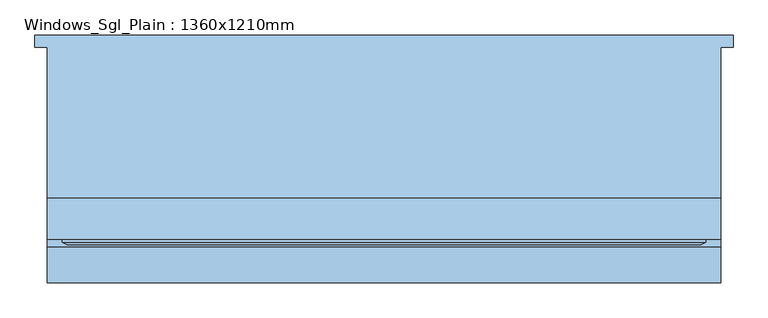
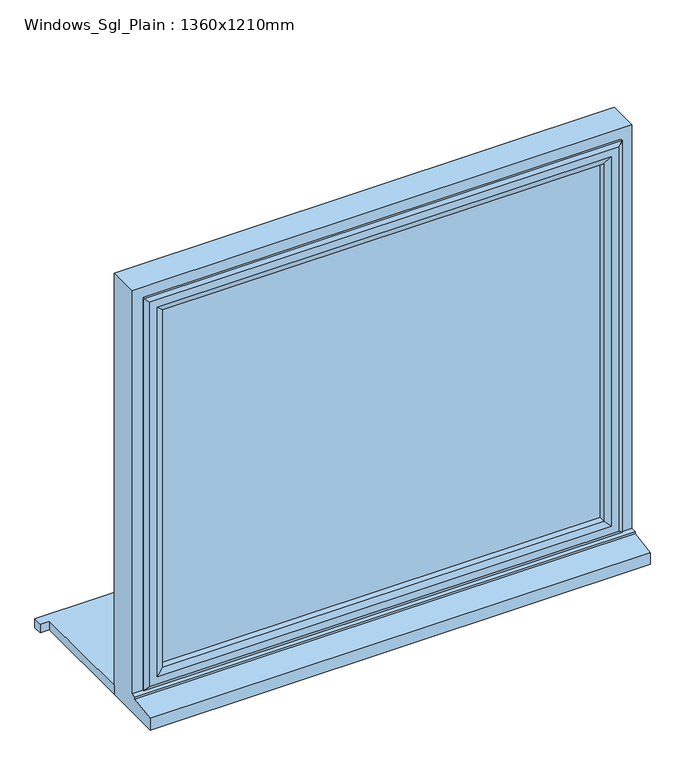
"""IFC4 building model written with IfcOpenShell, lengths in millimetres: window geometry, Windows_Sgl_Plain : 1360x1210mm."""

from ifc_helpers import new_model, si_unit, frame, origin, place, context, project, spatial, polyline, outline, extrude, faceted_brep, source, transform, mapped, element, save


def windows_sgl_plain_1360x1210mm_1c3d26f0(model_context):
    return source(origin(), model_context, "Body", "SolidModel", [
        extrude(outline(polyline([(-705.0, 235.2934322), (705.0, 235.2934322), (705.0, 210.2934322), (680.0, 210.2934322), (680.0, -94.2065678), (-680.0, -94.2065678), (-680.0, 210.2934322), (-705.0, 210.2934322), (-705.0, 235.2934322)])), frame((0.0, 0.0, 900.0), z_axis=(0.0, 0.0, 1.0), x_axis=(1.0, 0.0, 0.0)), (0.0, 0.0, 1.0), 25.0),
        faceted_brep([(-680.0, -94.2065678, 900.0), (-680.0, -94.2065678, 2110.0), (680.0, -94.2065678, 2110.0), (680.0, -94.2065678, 900.0), (-620.0, -94.2065678, 2050.0), (-620.0, -94.2065678, 975.0), (620.0, -94.2065678, 975.0), (620.0, -94.2065678, 2050.0), (-680.0, -264.7065678, 900.0), (-680.0, -264.7065678, 933.8088847), (-680.0, -192.2065678, 944.7449676), (-680.0, -192.2065678, 949.68767), (-680.0, -177.2065678, 951.0), (-680.0, -177.2065678, 2110.0), (680.0, -177.2065678, 951.0), (680.0, -177.2065678, 2110.0), (-640.0, -177.2065678, 2070.0), (640.0, -177.2065678, 2070.0), (640.0, -177.2065678, 963.0), (-640.0, -177.2065678, 963.0), (-640.0, -112.2065678, 963.0), (-640.0, -112.2065678, 2070.0), (640.0, -112.2065678, 963.0), (640.0, -112.2065678, 2070.0), (-620.0, -112.2065678, 2050.0), (620.0, -112.2065678, 2050.0), (620.0, -112.2065678, 975.0), (-620.0, -112.2065678, 975.0), (680.0, -192.2065678, 949.68767), (680.0, -192.2065678, 944.7449676), (680.0, -264.7065678, 933.8088847), (680.0, -264.7065678, 900.0)], [[[0, 1, 2, 3], [4, 5, 6, 7]], [[0, 8, 9, 10, 11, 12, 13, 1]], [[12, 14, 15, 13], [16, 17, 18, 19]], [[19, 20, 21, 16]], [[21, 20, 22, 23], [24, 25, 26, 27]], [[24, 27, 5, 4]], [[1, 13, 15, 2]], [[16, 21, 23, 17]], [[7, 25, 24, 4]], [[14, 28, 29, 30, 31, 3, 2, 15]], [[17, 23, 22, 18]], [[7, 6, 26, 25]], [[31, 8, 0, 3]], [[30, 9, 8, 31]], [[29, 10, 9, 30]], [[28, 11, 10, 29]], [[14, 12, 11, 28]], [[20, 19, 18, 22]], [[5, 27, 26, 6]]]),
        extrude(outline(polyline([(610.0, -141.2065678), (610.0, -165.2065678), (-610.0, -165.2065678), (-610.0, -141.2065678), (610.0, -141.2065678)])), frame((0.0, 0.0, 993.0), z_axis=(0.0, 0.0, 1.0), x_axis=(1.0, 0.0, 0.0)), (0.0, 0.0, 1.0), 1047.0),
        faceted_brep([(-650.0, -177.2065678, 2080.0), (-650.0, -177.2065678, 953.0), (-650.0, -182.9800705, 953.0), (-650.0, -182.9800705, 2080.0), (-640.0, -112.2065678, 2070.0), (-640.0, -112.2065678, 963.0), (-640.0, -177.2065678, 963.0), (-640.0, -177.2065678, 2070.0), (-600.0, -126.6994677, 2030.0), (-600.0, -126.6994677, 1003.0), (-610.1480377, -112.2065678, 992.8519623), (-610.1480377, -112.2065678, 2040.1480377), (-600.0, -141.2065678, 2030.0), (-600.0, -141.2065678, 1003.0), (-610.0, -165.2065678, 2040.0), (-610.0, -165.2065678, 993.0), (-610.0, -141.2065678, 993.0), (-610.0, -141.2065678, 2040.0), (-600.0, -182.9800705, 2030.0), (-600.0, -182.9800705, 1003.0), (-600.0, -165.2065678, 1003.0), (-600.0, -165.2065678, 2030.0), (-617.4457548, -188.7535732, 2047.4457548), (-617.4457548, -188.7535732, 985.5542452), (-639.2153903, -188.7535732, 963.7846097), (-639.2153903, -188.7535732, 2069.2153903), (650.0, -177.2065678, 953.0), (650.0, -182.9800705, 953.0), (640.0, -112.2065678, 963.0), (640.0, -177.2065678, 963.0), (600.0, -126.6994677, 1003.0), (610.1480377, -112.2065678, 992.8519623), (600.0, -141.2065678, 1003.0), (610.0, -165.2065678, 993.0), (610.0, -141.2065678, 993.0), (600.0, -182.9800705, 1003.0), (600.0, -165.2065678, 1003.0), (617.4457548, -188.7535732, 985.5542452), (639.2153903, -188.7535732, 963.7846097), (650.0, -177.2065678, 2080.0), (650.0, -182.9800705, 2080.0), (640.0, -112.2065678, 2070.0), (640.0, -177.2065678, 2070.0), (600.0, -126.6994677, 2030.0), (610.1480377, -112.2065678, 2040.1480377), (600.0, -141.2065678, 2030.0), (610.0, -165.2065678, 2040.0), (610.0, -141.2065678, 2040.0), (600.0, -182.9800705, 2030.0), (600.0, -165.2065678, 2030.0), (617.4457548, -188.7535732, 2047.4457548), (639.2153903, -188.7535732, 2069.2153903)], [[[0, 1, 2, 3]], [[4, 5, 6, 7]], [[8, 9, 10, 11]], [[12, 13, 9, 8]], [[14, 15, 16, 17]], [[18, 19, 20, 21]], [[22, 23, 19, 18]], [[3, 2, 24, 25]], [[1, 26, 27, 2]], [[5, 28, 29, 6]], [[9, 30, 31, 10]], [[13, 32, 30, 9]], [[15, 33, 34, 16]], [[19, 35, 36, 20]], [[23, 37, 35, 19]], [[2, 27, 38, 24]], [[26, 39, 40, 27]], [[28, 41, 42, 29]], [[30, 43, 44, 31]], [[32, 45, 43, 30]], [[33, 46, 47, 34]], [[35, 48, 49, 36]], [[37, 50, 48, 35]], [[27, 40, 51, 38]], [[39, 0, 3, 40]], [[1, 0, 39, 26], [7, 6, 29, 42]], [[41, 4, 7, 42]], [[5, 4, 41, 28], [11, 10, 31, 44]], [[43, 8, 11, 44]], [[45, 12, 8, 43]], [[17, 16, 34, 47], [13, 12, 45, 32]], [[46, 14, 17, 47]], [[15, 14, 46, 33], [21, 20, 36, 49]], [[48, 18, 21, 49]], [[50, 22, 18, 48]], [[25, 24, 38, 51], [23, 22, 50, 37]], [[40, 3, 25, 51]]]),
    ])


if __name__ == "__main__":
    model = new_model("IFC4")
    model_context = context("Model", 3, world=origin())
    ifc_project = project(units=[si_unit("LENGTHUNIT", "METRE", prefix="MILLI")], contexts=[model_context])
    site = spatial("IfcSite", under=ifc_project)
    building = spatial("IfcBuilding", under=site)
    placement = place(None, origin())
    windows_sgl_plain_1360x1210mm_shape = windows_sgl_plain_1360x1210mm_1c3d26f0(model_context)
    element("IfcWindow", 1, ObjectType="Windows_Sgl_Plain : 1360x1210mm", at=placement, inside=building, context=model_context, shape_type="MappedRepresentation", body=[
        mapped(windows_sgl_plain_1360x1210mm_shape, transform((0.0, 0.0, 0.0), x_axis=(1.0, 0.0, 0.0), y_axis=(0.0, 1.0, 0.0), z_axis=(0.0, 0.0, 1.0))),
    ])
    save(model, "model.ifc")

# Revit data of these elements
# Type "Windows_Sgl_Plain : 1360x1210mm"
#   Type Mark = "47"
#   Operation = "SinglePanel"
#   Construction Type Id = "SGL"
#   Manufacturer = "Revit"
#   Keynote = "L10"
#   Analytic Construction = "Large single-glazed windows"
#   Wrap Layers (Ext) from Ext = 102.5 mm
#   Wrap Layers (Int) from Ext = 177.5 mm
#   Window Board Projection = 25 mm
#   Window Board Extension = 25 mm
#   Visual Light Transmittance = 0.9
#   Solar Heat Gain Coefficient = 0.86
#   Rough Width = 1360 mm
#   Rough Height = 1210 mm
#   Height = 1210 mm
#   Width = 1360 mm
#   Heat Transfer Coefficient (U) = 5.5617 W/(m²·K)
#   Glazing Thickness = 24 mm
#   FrameOffset - External = 50 mm
#   Frame Depth = 65 mm
#   Default Head Height = 2110 mm
#   Cill Depth = 87.5 mm
#   Cavity Closer Width = 50 mm
#   Cavity Closer Offset from Ext = 102.5 mm
#   Cavity Closer Depth = 85 mm
#   Vis - Cavity Closers = yes
#   Material Trim = Window Frame
#   Material Glass = Glass
#   Material Frame = Window Frame
#   Wall Closure = (empty or 0)
# Element 1 (IfcWindow, "Windows_Sgl_Plain : 1360x1210mm")
#   Materials on its faces: "Window Frame", "Glass"
# Materials
#   "Window Frame": class "Miscellaneous", colour RGB 249 249 249, transparency 0, Keynote = "L10"
#   "Glass": class "Glass", colour RGB 0 128 192, transparency 0.9, Description = "Soda Lime Glass", Cost = 0
